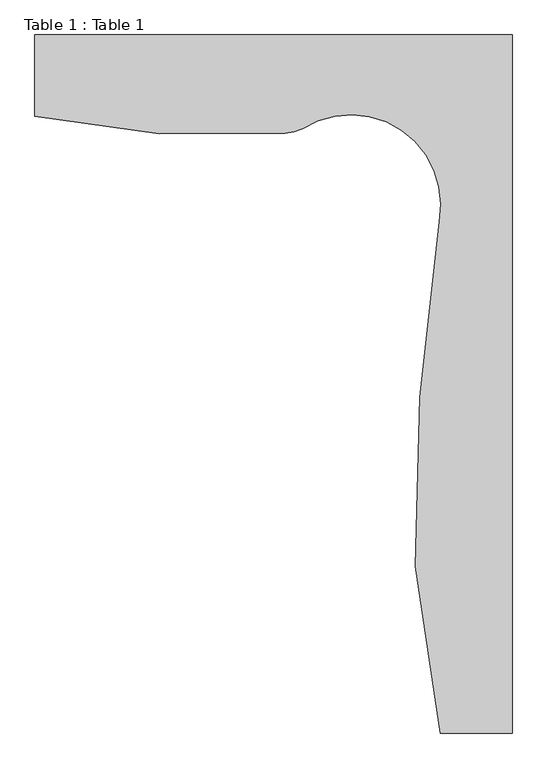
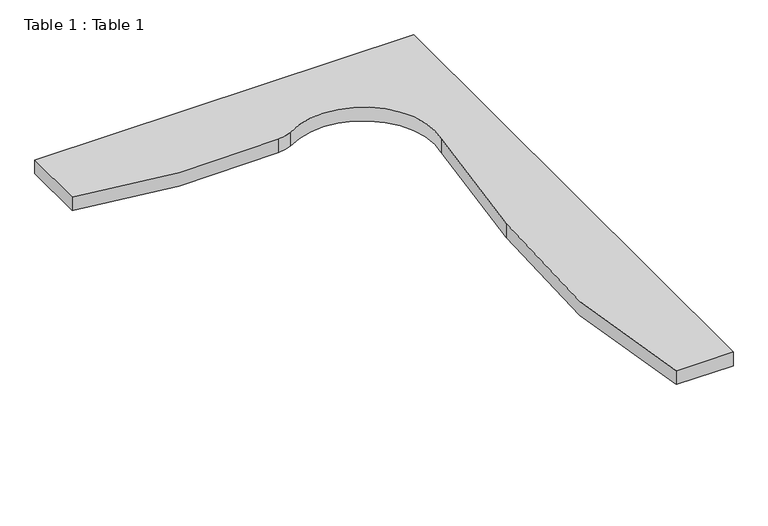
"""IFC4 building model written with IfcOpenShell, lengths in millimetres: furniture geometry, Table 1 : Table 1."""

import ifcopenshell
import ifcopenshell.guid

model = None  # the IFC model being written
_history = None  # IfcOwnerHistory: only IFC2X3 demands one
_inside = {}  # id of a spatial element -> (the spatial element, [elements in it])
_under = {}  # id of a project, library or spatial element -> (it, [spatial elements below it])
_declared = {}  # id of a project -> (the project, [libraries it declares])
_typed = {}  # id of a type object -> (the type object, [elements of that type])
_made_of = {}  # id of a material, layer set ... -> (it, [elements and type objects made of it])


def new_model(schema):
    """Start an empty IFC model of exactly this schema.

    Asked for "IFC4X3", IfcOpenShell would pick the latest addendum, in which some entities
    have other attributes; the version numbers below select the first issue.
    IFC2X3 requires an IfcOwnerHistory on every rooted entity: one is made here for all.
    """
    global model, _history
    if schema == "IFC4X3":
        model = ifcopenshell.file(schema_version=(4, 3, 0, 0))
    else:
        model = ifcopenshell.file(schema=schema)
    _inside.clear()
    _under.clear()
    _declared.clear()
    _typed.clear()
    _made_of.clear()
    _history = None
    if model.schema == "IFC2X3":
        org = make("IfcOrganization", Name="unknown")
        user = make(
            "IfcPersonAndOrganization",
            ThePerson=make("IfcPerson", FamilyName="unknown"),
            TheOrganization=org,
        )
        app = make(
            "IfcApplication",
            ApplicationDeveloper=org,
            Version="unknown",
            ApplicationFullName="unknown",
            ApplicationIdentifier="unknown",
        )
        _history = make(
            "IfcOwnerHistory",
            OwningUser=user,
            OwningApplication=app,
            ChangeAction="ADDED",
            CreationDate=0,
        )
    return model


def make(cls, **values):
    """One entity of the class cls with the attributes given. An attribute that is None is left unset."""
    return model.create_entity(
        cls, **{name: value for name, value in values.items() if value is not None}
    )


def rooted(cls, **values):
    """An entity with a GlobalId (a new one), such as an element, a storey or a relation."""
    return make(cls, GlobalId=ifcopenshell.guid.new(), OwnerHistory=_history, **values)


def si_unit(unit_type, name, prefix=None):
    """IfcSIUnit, for example si_unit("LENGTHUNIT", "METRE", prefix="MILLI")."""
    return make("IfcSIUnit", UnitType=unit_type, Prefix=prefix, Name=name)


def assignment(units):
    """IfcUnitAssignment: the units of a project."""
    return None if units is None else make("IfcUnitAssignment", Units=units)


def point(xyz):
    """IfcCartesianPoint."""
    return None if xyz is None else make("IfcCartesianPoint", Coordinates=xyz)


def direction(xyz):
    """IfcDirection."""
    return None if xyz is None else make("IfcDirection", DirectionRatios=xyz)


def frame(location, z_axis=None, x_axis=None):
    """IfcAxis2Placement3D, a coordinate frame: its origin and axes. An axis left out is left unset."""
    return make(
        "IfcAxis2Placement3D",
        Location=point(location),
        Axis=direction(z_axis),
        RefDirection=direction(x_axis),
    )


def frame_2d(location, x_axis=None):
    """IfcAxis2Placement2D, a coordinate frame in the plane: its origin and x axis."""
    return make(
        "IfcAxis2Placement2D", Location=point(location), RefDirection=direction(x_axis)
    )


def origin():
    """The frame at (0, 0, 0) with its axes left unset."""
    return frame((0.0, 0.0, 0.0))


def place(relative_to, where):
    """IfcLocalPlacement: puts the frame where relative to a parent placement (None: the world)."""
    return make(
        "IfcLocalPlacement", PlacementRelTo=relative_to, RelativePlacement=where
    )


def context(
    kind, dimensions, precision=None, world=None, true_north=None, identifier=None
):
    """IfcGeometricRepresentationContext, for example the 3D "Model" context."""
    return make(
        "IfcGeometricRepresentationContext",
        ContextIdentifier=identifier,
        ContextType=kind,
        CoordinateSpaceDimension=dimensions,
        Precision=precision,
        WorldCoordinateSystem=world,
        TrueNorth=true_north,
    )


def project(units=None, contexts=None):
    """IfcProject with its units and contexts."""
    return rooted(
        "IfcProject",
        Name="project",
        RepresentationContexts=contexts,
        UnitsInContext=assignment(units),
    )


def spatial(cls, under=None, at=None, **own):
    """A site, building, storey or space (cls), placed at a placement, below another one or the project."""
    s = rooted(cls, ObjectPlacement=at, **own)
    if under is not None:
        _under.setdefault(under.id(), (under, []))[1].append(s)
    return s


def polyline(points):
    """IfcPolyline through the points."""
    return make("IfcPolyline", Points=[point(p) for p in points])


def circle_curve(where, radius):
    """IfcCircle in the frame where."""
    return make("IfcCircle", Position=where, Radius=radius)


def trimmed(basis, trim1, trim2, sense, master):
    """IfcTrimmedCurve: the piece of a basis curve between two trims."""
    return make(
        "IfcTrimmedCurve",
        BasisCurve=basis,
        Trim1=trim1,
        Trim2=trim2,
        SenseAgreement=sense,
        MasterRepresentation=master,
    )


def segment(curve, same_sense, transition):
    """IfcCompositeCurveSegment."""
    return make(
        "IfcCompositeCurveSegment",
        Transition=transition,
        SameSense=same_sense,
        ParentCurve=curve,
    )


def composite_curve(segments, self_intersect=None):
    """IfcCompositeCurve: segments joined end to end."""
    return make("IfcCompositeCurve", Segments=segments, SelfIntersect=self_intersect)


def outline(outer, holes=None, kind="AREA"):
    """IfcArbitraryClosedProfileDef: a profile drawn as a closed curve; with holes, ...WithVoids."""
    if holes is None:
        return make("IfcArbitraryClosedProfileDef", ProfileType=kind, OuterCurve=outer)
    return make(
        "IfcArbitraryProfileDefWithVoids",
        ProfileType=kind,
        OuterCurve=outer,
        InnerCurves=holes,
    )


def extrude(swept, where, along, depth):
    """IfcExtrudedAreaSolid: the profile swept, set in the frame where, extruded along a direction by depth."""
    return make(
        "IfcExtrudedAreaSolid",
        SweptArea=swept,
        Position=where,
        ExtrudedDirection=direction(along),
        Depth=depth,
    )


def shape(context_of_items, identifier, shape_type, items):
    """IfcShapeRepresentation: the items that make up one representation, for example the "Body"."""
    return make(
        "IfcShapeRepresentation",
        ContextOfItems=context_of_items,
        RepresentationIdentifier=identifier,
        RepresentationType=shape_type,
        Items=items,
    )


def source(mapping_origin, context_of_items, identifier, shape_type, items):
    """IfcRepresentationMap: a shape defined once, which mapped items show again and again."""
    return make(
        "IfcRepresentationMap",
        MappingOrigin=mapping_origin,
        MappedRepresentation=shape(context_of_items, identifier, shape_type, items),
    )


def transform(
    local_origin,
    x_axis=None,
    y_axis=None,
    z_axis=None,
    scale=None,
    scale2=None,
    scale3=None,
    uniform=True,
):
    """IfcCartesianTransformationOperator3D, or its non-uniform kind. x_axis, y_axis, z_axis: its Axis1, 2, 3."""
    if uniform:
        return make(
            "IfcCartesianTransformationOperator3D",
            Axis1=direction(x_axis),
            Axis2=direction(y_axis),
            LocalOrigin=point(local_origin),
            Scale=scale,
            Axis3=direction(z_axis),
        )
    return make(
        "IfcCartesianTransformationOperator3DnonUniform",
        Axis1=direction(x_axis),
        Axis2=direction(y_axis),
        LocalOrigin=point(local_origin),
        Scale=scale,
        Axis3=direction(z_axis),
        Scale2=scale2,
        Scale3=scale3,
    )


def mapped(mapping_source, mapping_target):
    """IfcMappedItem: shows the shape of a source again, moved by a transform."""
    return make(
        "IfcMappedItem", MappingSource=mapping_source, MappingTarget=mapping_target
    )


def made_of(thing, what):
    """Note that an element or type object is made of a material, layer set ...; save() writes the relation."""
    if what is not None:
        _made_of.setdefault(what.id(), (what, []))[1].append(thing)
    return thing


def element(
    cls,
    number,
    at=None,
    inside=None,
    cuts=None,
    type_object=None,
    material=None,
    context=None,
    identifier="Body",
    shape_type=None,
    held_by="IfcProductDefinitionShape",
    body=None,
    shapes=None,
    **own,
):
    """One element of the class cls, such as IfcWall. Its Tag is "e" and its number.

    at: its placement. inside: the storey or other place that contains it. cuts: it is an
    opening in that element (IfcRelVoidsElement). A single representation is given by context,
    identifier, shape_type and body (its items); several are given by shapes. held_by: the class
    of the entity that holds the representations. save() writes the other relations.
    """
    e = rooted(cls, Tag="e%d" % number, ObjectPlacement=at, **own)
    if body is not None:
        shapes = [shape(context, identifier, shape_type, body)]
    if shapes is not None:
        e.Representation = make(held_by, Representations=shapes)
    if inside is not None:
        _inside.setdefault(inside.id(), (inside, []))[1].append(e)
    if cuts is not None:
        rooted(
            "IfcRelVoidsElement", RelatingBuildingElement=cuts, RelatedOpeningElement=e
        )
    if type_object is not None:
        _typed.setdefault(type_object.id(), (type_object, []))[1].append(e)
    return made_of(e, material)


def aggregate(whole, parts):
    """IfcRelAggregates: a whole, such as a stair, and the parts it consists of."""
    return rooted("IfcRelAggregates", RelatingObject=whole, RelatedObjects=parts)


def save(model, path):
    """Write the relations noted so far, then the file.

    IfcRelAggregates (storeys below a building ...), IfcRelContainedInSpatialStructure (elements
    in a storey), IfcRelDefinesByType, IfcRelAssociatesMaterial and IfcRelDeclares: one each for
    every whole, place, type object, material and project.
    """
    for whole, parts in _under.values():
        aggregate(whole, parts)
    for where, things in _inside.values():
        rooted(
            "IfcRelContainedInSpatialStructure",
            RelatedElements=things,
            RelatingStructure=where,
        )
    for kind, things in _typed.values():
        rooted("IfcRelDefinesByType", RelatedObjects=things, RelatingType=kind)
    for what, things in _made_of.values():
        rooted("IfcRelAssociatesMaterial", RelatedObjects=things, RelatingMaterial=what)
    for by, libraries in _declared.values():
        rooted("IfcRelDeclares", RelatingContext=by, RelatedDefinitions=libraries)
    model.write(path)


def table_1_table_1_ccfc99bd(model_context):
    return source(origin(), model_context, "Body", "SweptSolid", [
        extrude(outline(composite_curve([segment(polyline([(-1445.9590575, 1770.3451612), (-1445.9590575, 2215.345166), (1167.9773926, 2215.345166), (1167.9773926, -1605.8191519), (775.2013102, -1605.8191519)]), True, "CONTINUOUS"), segment(trimmed(circle_curve(frame_2d((5888.8305414, -371.2496725)), 5260.5480431), [point((775.2013102, -1605.8191519))], [point((662.9577661, 231.758993))], False, "CARTESIAN"), True, "CONTINUOUS"), segment(trimmed(circle_curve(frame_2d((7623.8618479, -51.0644744)), 6966.6473106), [point((662.9577661, 231.758993))], [point((769.2336036, 1193.221016))], False, "CARTESIAN"), True, "CONTINUOUS"), segment(trimmed(circle_curve(frame_2d((285.1539356, 1285.754003)), 492.8442742), [point((769.2336036, 1193.221016))], [point((20.9499867, 1701.796972))], True, "CARTESIAN"), True, "CONTINUOUS"), segment(trimmed(circle_curve(frame_2d((-96.9053466, 1964.964372)), 288.3521459), [point((20.9499867, 1701.796972))], [point((-74.9606604, 1677.4484754))], False, "CARTESIAN"), True, "CONTINUOUS"), segment(trimmed(circle_curve(frame_2d((-445.9066277, 6366.1719672)), 4703.3742029), [point((-74.9606604, 1677.4484754))], [point((-1445.9590575, 1770.3451612))], False, "CARTESIAN"), True, "CONTINUOUS")], self_intersect=False)), frame((0.0, 0.0, 600.0), z_axis=(0.0, 0.0, 1.0), x_axis=(1.0, 0.0, 0.0)), (0.0, 0.0, 1.0), 100.0),
    ])


if __name__ == "__main__":
    model = new_model("IFC4")
    model_context = context("Model", 3, world=origin())
    ifc_project = project(units=[si_unit("LENGTHUNIT", "METRE", prefix="MILLI")], contexts=[model_context])
    site = spatial("IfcSite", under=ifc_project)
    building = spatial("IfcBuilding", under=site)
    placement = place(None, origin())
    table_1_table_1_shape = table_1_table_1_ccfc99bd(model_context)
    element("IfcFurniture", 1, ObjectType="Table 1 : Table 1", at=placement, inside=building, context=model_context, shape_type="MappedRepresentation", body=[
        mapped(table_1_table_1_shape, transform((0.0, 0.0, 0.0), x_axis=(1.0, 0.0, 0.0), y_axis=(0.0, 1.0, 0.0), z_axis=(0.0, 0.0, 1.0))),
    ])
    save(model, "model.ifc")

# Revit data of these elements
# Type "Table 1 : Table 1"
#   COBie.Type.CreatedBy = "design@eagle.com"
#   COBie.Type.CreatedOn = "2016-09-13T05:47:35"
#   COBie.Type.Name = "Furniture Systems_Table 1_Table 1"
#   COBie.Type.Category = "23-40 70 14 64 21 21 : Desk System"
#   COBie.Type.Description = ""
#   COBie.Type.Manufacturer = ""
#   COBie.Type.ModelNumber = ""
#   COBie.Type.ReplacementCost = 0
#   COBie.Type = yes
